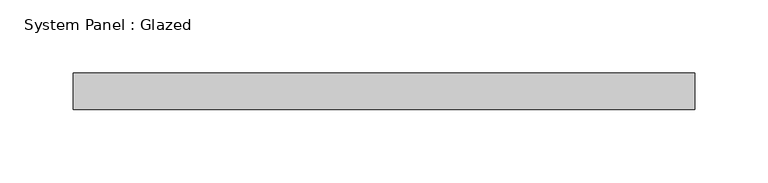
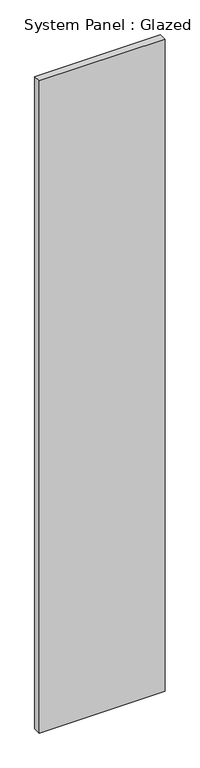
"""IFC4 building model written with IfcOpenShell, lengths in millimetres: plate geometry, System Panel : Glazed."""

from ifc_helpers import new_model, si_unit, origin, origin_with_axes, place, context, project, spatial, polyline, outline, extrude, source, transform, mapped, element, save


def system_panel_glazed_bbee96c2(model_context):
    return source(origin(), model_context, "Body", "SweptSolid", [
        extrude(outline(polyline([(212.5000001, 24.5), (-212.5000001, 24.5), (-212.5000001, 49.5), (212.5000001, 49.5), (212.5000001, 24.5)])), origin_with_axes(), (0.0, 0.0, 1.0), 2325.0),
    ])


if __name__ == "__main__":
    model = new_model("IFC4")
    model_context = context("Model", 3, world=origin())
    ifc_project = project(units=[si_unit("LENGTHUNIT", "METRE", prefix="MILLI")], contexts=[model_context])
    site = spatial("IfcSite", under=ifc_project)
    building = spatial("IfcBuilding", under=site)
    placement = place(None, origin())
    system_panel_glazed_shape = system_panel_glazed_bbee96c2(model_context)
    element("IfcPlate", 1, ObjectType="System Panel : Glazed", at=placement, inside=building, context=model_context, shape_type="MappedRepresentation", body=[
        mapped(system_panel_glazed_shape, transform((0.0, 0.0, 0.0), x_axis=(1.0, 0.0, 0.0), y_axis=(0.0, 1.0, 0.0), z_axis=(0.0, 0.0, 1.0))),
    ])
    save(model, "model.ifc")

# Revit data of these elements
# Type "System Panel : Glazed"
#   Construction Type Id = "GSP4R"
#   Analytic Construction = "1/8 in Pilkington single glazing"
#   Visual Light Transmittance = 0.9
#   Solar Heat Gain Coefficient = 0.86
#   Heat Transfer Coefficient (U) = 6.7069 W/(m²·K)
#   Define Thermal Properties by = 1
# Element 1 (IfcPlate, "System Panel : Glazed")
#   Materials on its faces: "Glass"
# Materials
#   "Glass": class "Glass", colour RGB 0 128 192, transparency 0.9, Description = "Soda Lime Glass", Cost = 0
